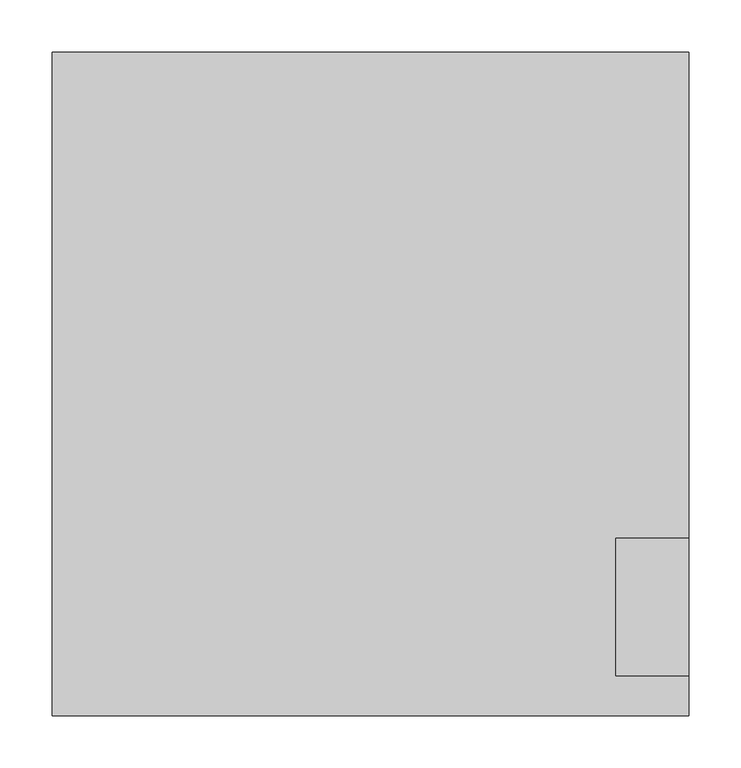
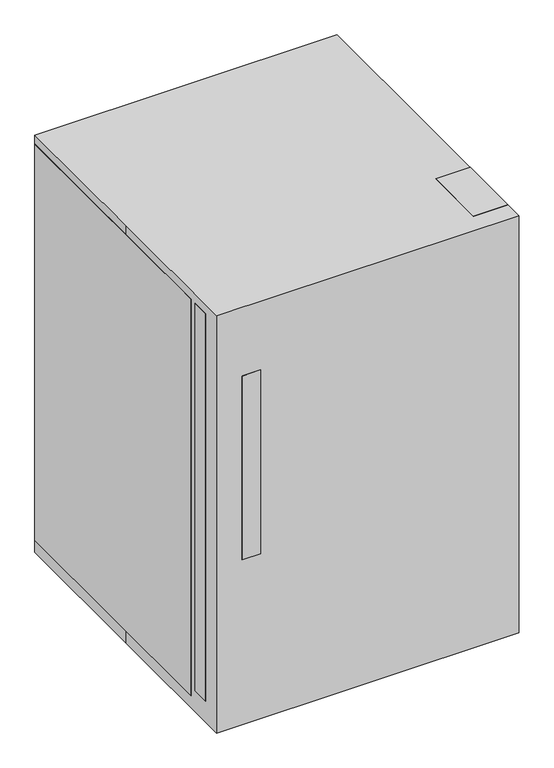
"""IFC4 building model written with IfcOpenShell, lengths in millimetres: proxy geometry, R6200 - Refrigerator, U-C or F-S, 5 Cu Ft : R6200 - Refrigerator, U-C or F-S, 5 Cu Ft."""

from ifc_helpers import new_model, si_unit, point, frame, frame_2d, origin, origin_with_axes, place, context, project, spatial, polyline, circle_curve, trimmed, segment, composite_curve, outline, extrude, source, transform, mapped, element, save


def specialty_equipment_522e98b9(model_context):
    return source(origin(), model_context, "Body", "SweptSolid", [
        extrude(outline(polyline([(304.8, -279.4), (234.95, -279.4), (234.95, -228.6), (304.8, -228.6), (304.8, -279.4)])), frame((0.0, 0.0, 25.4), z_axis=(0.0, 0.0, 1.0), x_axis=(1.0, 0.0, 0.0)), (0.0, 0.0, 1.0), 19.05),
        extrude(outline(polyline([(-317.5, 351.4614039), (-317.5, 742.95), (-279.4, 742.95), (-279.4, 730.2659299), (-304.8159299, 730.2659299), (-304.8159299, 364.1614039), (-279.4, 364.1614039), (-279.4, 351.4614039), (-317.5, 351.4614039)])), frame((-254.0, 0.0, 0.0), z_axis=(1.0, 0.0, 0.0), x_axis=(0.0, 1.0, 0.0)), (0.0, 0.0, 1.0), 38.1),
        extrude(outline(polyline([(304.8, -279.4), (234.95, -279.4), (234.95, -147.9315495), (304.8, -147.9315495), (304.8, -279.4)])), frame((0.0, 0.0, 869.95), z_axis=(0.0, 0.0, 1.0), x_axis=(1.0, 0.0, 0.0)), (0.0, 0.0, 1.0), 19.05),
        extrude(outline(polyline([(292.1, -241.3), (-292.1, -241.3), (-292.1, -228.6), (292.1, -228.6), (292.1, -241.3)])), frame((0.0, 0.0, 66.7735467), z_axis=(0.0, 0.0, 1.0), x_axis=(1.0, 0.0, 0.0)), (0.0, 0.0, 1.0), 771.4264533),
        extrude(outline(polyline([(304.8, -279.4), (-304.8, -279.4), (-304.8, -241.3), (304.8, -241.3), (304.8, -279.4)])), frame((0.0, 0.0, 44.45), z_axis=(0.0, 0.0, 1.0), x_axis=(1.0, 0.0, 0.0)), (0.0, 0.0, 1.0), 825.5),
        extrude(outline(polyline([(304.8, 317.5), (304.8, -228.6), (-304.8, -228.6), (-304.8, 317.5), (304.8, 317.5)])), frame((0.0, 0.0, 25.4), z_axis=(0.0, 0.0, 1.0), x_axis=(1.0, 0.0, 0.0)), (0.0, 0.0, 1.0), 844.55),
        extrude(outline(composite_curve([segment(trimmed(circle_curve(frame_2d((-231.6775617, -167.1820241)), 31.75), [point((-199.9275617, -167.1820241))], [point((-263.4275617, -167.1820241))], False, "CARTESIAN"), True, "CONTINUOUS"), segment(trimmed(circle_curve(frame_2d((-231.6775617, -167.1820241)), 31.75), [point((-263.4275617, -167.1820241))], [point((-199.9275617, -167.1820241))], False, "CARTESIAN"), True, "CONTINUOUS")], self_intersect=False)), origin_with_axes(), (0.0, 0.0, 1.0), 25.4),
        extrude(outline(composite_curve([segment(trimmed(circle_curve(frame_2d((231.6775617, -167.1820241)), 31.75), [point((199.9275617, -167.1820241))], [point((263.4275617, -167.1820241))], False, "CARTESIAN"), True, "CONTINUOUS"), segment(trimmed(circle_curve(frame_2d((231.6775617, -167.1820241)), 31.75), [point((263.4275617, -167.1820241))], [point((199.9275617, -167.1820241))], False, "CARTESIAN"), True, "CONTINUOUS")], self_intersect=False)), origin_with_axes(), (0.0, 0.0, 1.0), 25.4),
        extrude(outline(composite_curve([segment(trimmed(circle_curve(frame_2d((-231.6775617, 251.9179759)), 31.75), [point((-199.9275617, 251.9179759))], [point((-263.4275617, 251.9179759))], False, "CARTESIAN"), True, "CONTINUOUS"), segment(trimmed(circle_curve(frame_2d((-231.6775617, 251.9179759)), 31.75), [point((-263.4275617, 251.9179759))], [point((-199.9275617, 251.9179759))], False, "CARTESIAN"), True, "CONTINUOUS")], self_intersect=False)), origin_with_axes(), (0.0, 0.0, 1.0), 25.4),
        extrude(outline(composite_curve([segment(trimmed(circle_curve(frame_2d((231.6775617, 251.9179759)), 31.75), [point((199.9275617, 251.9179759))], [point((263.4275617, 251.9179759))], False, "CARTESIAN"), True, "CONTINUOUS"), segment(trimmed(circle_curve(frame_2d((231.6775617, 251.9179759)), 31.75), [point((263.4275617, 251.9179759))], [point((199.9275617, 251.9179759))], False, "CARTESIAN"), True, "CONTINUOUS")], self_intersect=False)), origin_with_axes(), (0.0, 0.0, 1.0), 25.4),
        extrude(outline(polyline([(-304.8, 317.5), (304.8, 317.5), (304.8, -317.5), (-304.8, -317.5), (-304.8, 0.0), (-304.8, 317.5)])), origin_with_axes(), (0.0, 0.0, 1.0), 889.0),
    ])


if __name__ == "__main__":
    model = new_model("IFC4")
    model_context = context("Model", 3, world=origin())
    ifc_project = project(units=[si_unit("LENGTHUNIT", "METRE", prefix="MILLI")], contexts=[model_context])
    site = spatial("IfcSite", under=ifc_project)
    building = spatial("IfcBuilding", under=site)
    placement = place(None, origin())
    specialty_equipment_shape = specialty_equipment_522e98b9(model_context)
    element("IfcBuildingElementProxy", 1, Name="R6200 - Refrigerator, U-C or F-S, 5 Cu Ft : R6200 - Refrigerator, U-C or F-S, 5 Cu Ft", ObjectType="R6200 - Refrigerator, U-C or F-S, 5 Cu Ft : R6200 - Refrigerator, U-C or F-S, 5 Cu Ft", at=placement, inside=building, context=model_context, shape_type="MappedRepresentation", body=[
        mapped(specialty_equipment_shape, transform((0.0, 0.0, 0.0), x_axis=(1.0, 0.0, 0.0), y_axis=(0.0, 1.0, 0.0), z_axis=(0.0, 0.0, 1.0))),
    ])
    save(model, "model.ifc")

# Revit data of these elements
# Project information
#   Sheets - Total = "5"
#   Project Issue Date = "Issue Date"
#   Project Status = "Project Status"
#   Client Name = "Owner"
#   Project Address = "Enter address here"
#   Project Name = "Project Name"
#   Project Number = "Project Number"
#   Publication Date = "30-Jan-15"
# Type "R6200 - Refrigerator, U-C or F-S, 5 Cu Ft : R6200 - Refrigerator, U-C or F-S, 5 Cu Ft"
#   Watts2 = "0"
#   Watts1 = "480"
#   Unit_Issue = "EA"
#   UTIL_6_Misc = "-"
#   UTIL_5_NonMedGas = "-"
#   UTIL_4_MiscGas = "-"
#   UTIL_3_MedGas = "-"
#   UTIL_2_Elec = "A"
#   UTIL_1_WaterDrain = "-"
#   Nomenclature = "Refrigerator, U/C or F/S, 5 Cu Ft"
#   NSN = "4110"
#   Location [instance default] = ""
#   JSN = "R6200"
#   Fund_Source_VA = "-"
#   Fund_Source_Navy = "-"
#   Fund_Source_Army = "-"
#   Fund_Source_AF = "-"
#   ELEC_Volts2 = "0"
#   ELEC_Volts1 = "120"
#   ELEC_Phase2 = "0"
#   ELEC_Phase1 = "1"
#   ELEC_HertzSwitch = "0"
#   ELEC_HertzDependent = "-1"
#   ELEC_Hertz = "60"
#   ELEC_Amps2 = "0"
#   ELEC_Amps1 = "4"
#   DetailDescription = "Utility refrigerator approximately 35\" H x 24\" W x 26\" D. The unit has a two tray ice cube cooling system. The refrigerator fits standard architectural dimensions for undercounter installation. The unit is perfect for use in nurses' station, wards, and laboratories, pharmacies or wherever space is limited."
#   CAT_VA = "C"
#   CAT_Navy = "C"
#   CAT_IHS = "-"
#   CAT_Army = "C"
#   CAT_AF = "C"
#   BTUperhour = "900"
#   Weight_IP = 120
#   DIM_Width_IP = 2' - 0"
#   DIM_Height_IP = 2' - 11"
#   DIM_Depth_IP = 2' - 1"
# Element 1 (IfcBuildingElementProxy, "R6200 - Refrigerator, U-C or F-S, 5 Cu Ft : R6200 - Refrigerator, U-C or F-S, 5 Cu Ft")
#   Materials on its faces: "EquipSpace"
# Materials
#   "EquipSpace": class "Unassigned", colour RGB 221 217 195, transparency 0.5
